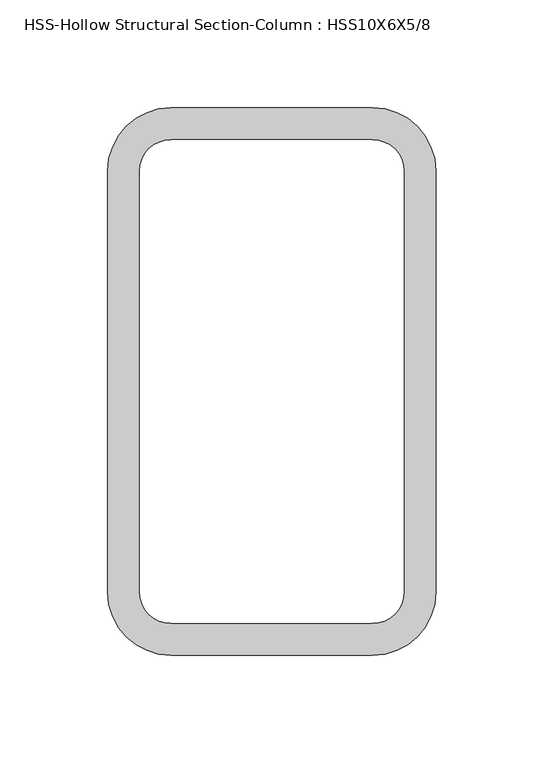
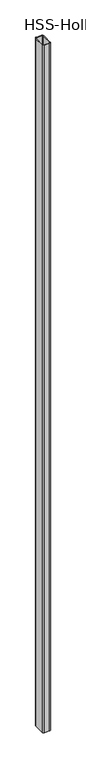
"""IFC4 building model written with IfcOpenShell, lengths in millimetres: column geometry, HSS-Hollow Structural Section-Column : HSS10X6X5/8."""

from ifc_helpers import new_model, si_unit, point, frame, frame_2d, origin, place, context, project, spatial, polyline, circle_curve, trimmed, segment, composite_curve, outline, extrude, source, transform, mapped, element, save


def hss_hollow_structural_section_column_hss10x6x5_8_25c5c677(model_context):
    return source(origin(), model_context, "Body", "SweptSolid", [
        extrude(outline(composite_curve([segment(trimmed(circle_curve(frame_2d((46.6852, 97.4852)), 29.5148), [point((46.6852, 127.0))], [point((76.2, 97.4852))], False, "CARTESIAN"), True, "CONTINUOUS"), segment(polyline([(76.2, 97.4852), (76.2, -97.4852)]), True, "CONTINUOUS"), segment(trimmed(circle_curve(frame_2d((46.6852, -97.4852)), 29.5148), [point((76.2, -97.4852))], [point((46.6852, -127.0))], False, "CARTESIAN"), True, "CONTINUOUS"), segment(polyline([(46.6852, -127.0), (-46.6852, -127.0)]), True, "CONTINUOUS"), segment(trimmed(circle_curve(frame_2d((-46.6852, -97.4852)), 29.5148), [point((-46.6852, -127.0))], [point((-76.2, -97.4852))], False, "CARTESIAN"), True, "CONTINUOUS"), segment(polyline([(-76.2, -97.4852), (-76.2, 97.4852)]), True, "CONTINUOUS"), segment(trimmed(circle_curve(frame_2d((-46.6852, 97.4852)), 29.5148), [point((-76.2, 97.4852))], [point((-46.6852, 127.0))], False, "CARTESIAN"), True, "CONTINUOUS"), segment(polyline([(-46.6852, 127.0), (46.6852, 127.0)]), True, "CONTINUOUS")], self_intersect=False), holes=[composite_curve([segment(polyline([(46.6852, 112.2426), (-46.6852, 112.2426)]), True, "CONTINUOUS"), segment(trimmed(circle_curve(frame_2d((-46.6852, 97.4852)), 14.7574), [point((-46.6852, 112.2426))], [point((-61.4426, 97.4852))], True, "CARTESIAN"), True, "CONTINUOUS"), segment(polyline([(-61.4426, 97.4852), (-61.4426, -97.4852)]), True, "CONTINUOUS"), segment(trimmed(circle_curve(frame_2d((-46.6852, -97.4852)), 14.7574), [point((-61.4426, -97.4852))], [point((-46.6852, -112.2426))], True, "CARTESIAN"), True, "CONTINUOUS"), segment(polyline([(-46.6852, -112.2426), (46.6852, -112.2426)]), True, "CONTINUOUS"), segment(trimmed(circle_curve(frame_2d((46.6852, -97.4852)), 14.7574), [point((46.6852, -112.2426))], [point((61.4426, -97.4852))], True, "CARTESIAN"), True, "CONTINUOUS"), segment(polyline([(61.4426, -97.4852), (61.4426, 97.4852)]), True, "CONTINUOUS"), segment(trimmed(circle_curve(frame_2d((46.6852, 97.4852)), 14.7574), [point((61.4426, 97.4852))], [point((46.6852, 112.2426))], True, "CARTESIAN"), True, "CONTINUOUS")], self_intersect=False)]), frame((0.0, 0.0, -609.6), z_axis=(0.0, 0.0, 1.0), x_axis=(1.0, 0.0, 0.0)), (0.0, 0.0, 1.0), 13157.2),
    ])


if __name__ == "__main__":
    model = new_model("IFC4")
    model_context = context("Model", 3, world=origin())
    ifc_project = project(units=[si_unit("LENGTHUNIT", "METRE", prefix="MILLI")], contexts=[model_context])
    site = spatial("IfcSite", under=ifc_project)
    building = spatial("IfcBuilding", under=site)
    placement = place(None, origin())
    hss_hollow_structural_section_column_hss10x6x5_8_shape = hss_hollow_structural_section_column_hss10x6x5_8_25c5c677(model_context)
    element("IfcColumn", 1, ObjectType="HSS-Hollow Structural Section-Column : HSS10X6X5/8", at=placement, inside=building, context=model_context, shape_type="MappedRepresentation", body=[
        mapped(hss_hollow_structural_section_column_hss10x6x5_8_shape, transform((0.0, 0.0, 0.0), x_axis=(1.0, 0.0, 0.0), y_axis=(0.0, 1.0, 0.0), z_axis=(0.0, 0.0, 1.0))),
    ])
    save(model, "model.ifc")

# Revit data of these elements
# Type "HSS-Hollow Structural Section-Column : HSS10X6X5/8"
#   Assembly Code = "B10"
#   Shape = "Rect."
#   W = 59.1
#   Ht = 0' - 10"
#   b = 0' - 6"
#   kr = 0' - 1.162"
#   t = 0' - 0.581"
#   A = 0.113889 SF
#   Structural Material [instance default] = Steel ASTM A500, Grade B, Rectangular and Square
# Element 1 (IfcColumn, "HSS-Hollow Structural Section-Column : HSS10X6X5/8")
#   Materials on its faces: "Steel ASTM A500, Grade B, Rectangular and Square"
# Materials
#   "Steel ASTM A500, Grade B, Rectangular and Square": class "Metal", colour RGB 199 199 199, transparency 0, Description = "Carbon steel", Cost = 0
